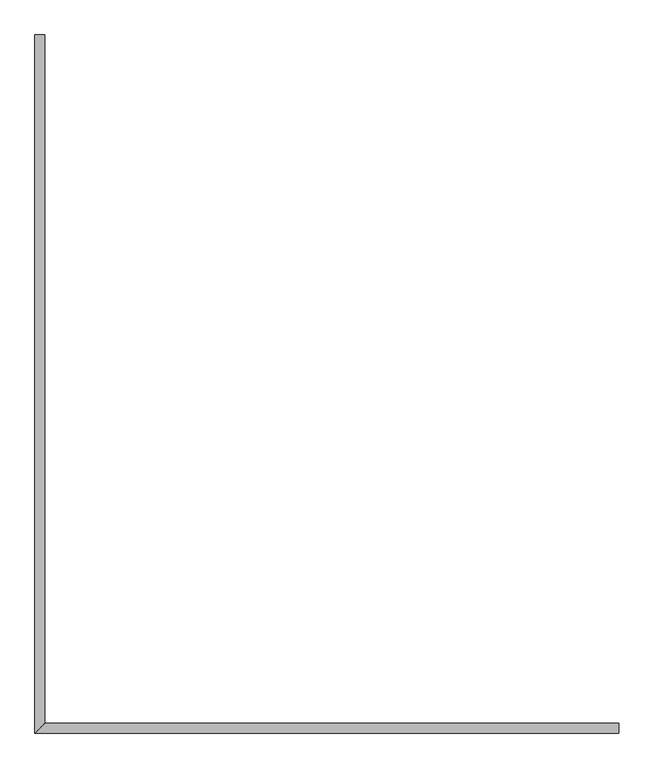
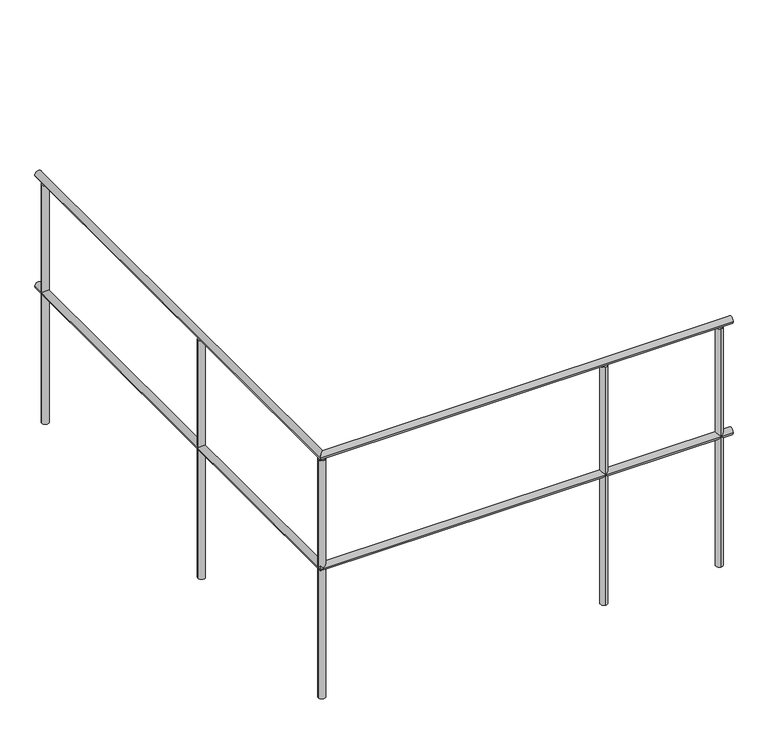
"""IFC4 building model written with IfcOpenShell, lengths in millimetres: railing geometry."""

from ifc_helpers import new_model, si_unit, point, frame, frame_2d, origin, place, context, project, spatial, circle_curve, ellipse_curve, trimmed, segment, composite_curve, outline, extrude, source, transform, mapped, element, save
from ifc_brep_helpers import plane_surface, cylinder_surface, advanced_brep


def railing_e5dc5f3b(model_context):
    return source(origin(), model_context, "Body", "SolidModel", [
        advanced_brep(
        [(-2206.0, 33046.2934796, 885.0), (-2176.0, 33046.2934796, 885.0), (-2176.0, 30976.2934796, 885.0), (-2206.0, 30946.2934796, 885.0), (-450.0, 30946.2934796, 885.0), (-450.0, 30976.2934796, 885.0)],
        [
            (0, 1, circle_curve(frame((-2191.0, 33046.2934796, 885.0), z_axis=(0.0, 1.0, 0.0), x_axis=(1.0, 0.0, 0.0)), 15.0)),
            (1, 0, circle_curve(frame((-2191.0, 33046.2934796, 885.0), z_axis=(0.0, 1.0, 0.0), x_axis=(1.0, 0.0, 0.0)), 15.0)),
            (1, 2),
            (2, 3, ellipse_curve(frame((-2191.0, 30961.2934796, 885.0), z_axis=(-0.707106781186546, 0.707106781186549, 0.0), x_axis=(0.7071067811865489, 0.707106781186546, 0.0)), 21.2132034, 15.0)),
            (3, 0),
            (3, 2, ellipse_curve(frame((-2191.0, 30961.2934796, 885.0), z_axis=(-0.707106781186546, 0.707106781186549, 0.0), x_axis=(0.7071067811865489, 0.707106781186546, 0.0)), 21.2132034, 15.0)),
            (4, 5, circle_curve(frame((-450.0, 30961.2934796, 885.0), z_axis=(1.0, 0.0, 0.0), x_axis=(0.0, 1.0, 0.0)), 15.0)),
            (5, 4, circle_curve(frame((-450.0, 30961.2934796, 885.0), z_axis=(1.0, 0.0, 0.0), x_axis=(0.0, 1.0, 0.0)), 15.0)),
            (2, 5),
            (4, 3),
        ],
        [
            plane_surface(frame((-2191.0, 33046.2934796, 900.0), z_axis=(0.0, 1.0, 0.0), x_axis=(0.0, 0.0, -1.0))),
            cylinder_surface(frame((-2191.0, 33046.2934796, 885.0), z_axis=(0.0, 1.0, 0.0), x_axis=(1.0, 0.0, 0.0)), 15.0),
            plane_surface(frame((-450.0, 30961.2934796, 900.0), z_axis=(1.0, 0.0, 0.0), x_axis=(0.0, 1.0, 0.0))),
            cylinder_surface(frame((-2191.0, 30961.2934796, 885.0), z_axis=(-1.0, 0.0, 0.0), x_axis=(0.0, 1.0, 0.0)), 15.0),
        ],
        [
            (0, [[1, 2]]),
            (1, [[-2, 3, 4, 5]]),
            (1, [[-1, -5, 6, -3]]),
            (2, [[7, 8]]),
            (3, [[-4, 9, -7, 10]]),
            (3, [[-6, -10, -8, -9]]),
        ],
    ),
        advanced_brep(
        [(-2206.0, 33046.2934796, 1385.0), (-2176.0, 33046.2934796, 1385.0), (-2176.0, 30976.2934796, 1385.0), (-2206.0, 30946.2934796, 1385.0), (-450.0, 30946.2934796, 1385.0), (-450.0, 30976.2934796, 1385.0)],
        [
            (0, 1, circle_curve(frame((-2191.0, 33046.2934796, 1385.0), z_axis=(0.0, 1.0, 0.0), x_axis=(1.0, 0.0, 0.0)), 15.0)),
            (1, 0, circle_curve(frame((-2191.0, 33046.2934796, 1385.0), z_axis=(0.0, 1.0, 0.0), x_axis=(1.0, 0.0, 0.0)), 15.0)),
            (1, 2),
            (2, 3, ellipse_curve(frame((-2191.0, 30961.2934796, 1385.0), z_axis=(-0.707106781186546, 0.707106781186549, 0.0), x_axis=(0.7071067811865489, 0.707106781186546, 0.0)), 21.2132034, 15.0)),
            (3, 0),
            (3, 2, ellipse_curve(frame((-2191.0, 30961.2934796, 1385.0), z_axis=(-0.707106781186546, 0.707106781186549, 0.0), x_axis=(0.7071067811865489, 0.707106781186546, 0.0)), 21.2132034, 15.0)),
            (4, 5, circle_curve(frame((-450.0, 30961.2934796, 1385.0), z_axis=(1.0, 0.0, 0.0), x_axis=(0.0, 1.0, 0.0)), 15.0)),
            (5, 4, circle_curve(frame((-450.0, 30961.2934796, 1385.0), z_axis=(1.0, 0.0, 0.0), x_axis=(0.0, 1.0, 0.0)), 15.0)),
            (2, 5),
            (4, 3),
        ],
        [
            plane_surface(frame((-2191.0, 33046.2934796, 1400.0), z_axis=(0.0, 1.0, 0.0), x_axis=(0.0, 0.0, -1.0))),
            cylinder_surface(frame((-2191.0, 33046.2934796, 1385.0), z_axis=(0.0, 1.0, 0.0), x_axis=(1.0, 0.0, 0.0)), 15.0),
            plane_surface(frame((-450.0, 30961.2934796, 1400.0), z_axis=(1.0, 0.0, 0.0), x_axis=(0.0, 1.0, 0.0))),
            cylinder_surface(frame((-2191.0, 30961.2934796, 1385.0), z_axis=(-1.0, 0.0, 0.0), x_axis=(0.0, 1.0, 0.0)), 15.0),
        ],
        [
            (0, [[1, 2]]),
            (1, [[-2, 3, 4, 5]]),
            (1, [[-1, -5, 6, -3]]),
            (2, [[7, 8]]),
            (3, [[-4, 9, -7, 10]]),
            (3, [[-6, -10, -8, -9]]),
        ],
    ),
        extrude(outline(composite_curve([segment(trimmed(circle_curve(frame_2d((-991.0, 30961.2934796)), 15.0), [point((-991.0, 30946.2934796))], [point((-991.0, 30976.2934796))], False, "CARTESIAN"), True, "CONTINUOUS"), segment(trimmed(circle_curve(frame_2d((-991.0, 30961.2934796)), 15.0), [point((-991.0, 30976.2934796))], [point((-991.0, 30946.2934796))], False, "CARTESIAN"), True, "CONTINUOUS")], self_intersect=False)), frame((0.0, 0.0, 300.0), z_axis=(0.0, 0.0, 1.0), x_axis=(1.0, 0.0, 0.0)), (0.0, 0.0, 1.0), 1070.0),
        extrude(outline(composite_curve([segment(trimmed(circle_curve(frame_2d((-2191.0, 31846.2934796)), 15.0), [point((-2206.0, 31846.2934796))], [point((-2176.0, 31846.2934796))], False, "CARTESIAN"), True, "CONTINUOUS"), segment(trimmed(circle_curve(frame_2d((-2191.0, 31846.2934796)), 15.0), [point((-2176.0, 31846.2934796))], [point((-2206.0, 31846.2934796))], False, "CARTESIAN"), True, "CONTINUOUS")], self_intersect=False)), frame((0.0, 0.0, 300.0), z_axis=(0.0, 0.0, 1.0), x_axis=(1.0, 0.0, 0.0)), (0.0, 0.0, 1.0), 1070.0),
        extrude(outline(composite_curve([segment(trimmed(circle_curve(frame_2d((-2191.0, 30961.2934796)), 15.0), [point((-2206.0, 30961.2934796))], [point((-2176.0, 30961.2934796))], False, "CARTESIAN"), True, "CONTINUOUS"), segment(trimmed(circle_curve(frame_2d((-2191.0, 30961.2934796)), 15.0), [point((-2176.0, 30961.2934796))], [point((-2206.0, 30961.2934796))], False, "CARTESIAN"), True, "CONTINUOUS")], self_intersect=False)), frame((0.0, 0.0, 300.0), z_axis=(0.0, 0.0, 1.0), x_axis=(1.0, 0.0, 0.0)), (0.0, 0.0, 1.0), 1070.0),
        extrude(outline(composite_curve([segment(trimmed(circle_curve(frame_2d((-500.0, 30961.2934796)), 15.0), [point((-500.0, 30946.2934796))], [point((-500.0, 30976.2934796))], False, "CARTESIAN"), True, "CONTINUOUS"), segment(trimmed(circle_curve(frame_2d((-500.0, 30961.2934796)), 15.0), [point((-500.0, 30976.2934796))], [point((-500.0, 30946.2934796))], False, "CARTESIAN"), True, "CONTINUOUS")], self_intersect=False)), frame((0.0, 0.0, 300.0), z_axis=(0.0, 0.0, 1.0), x_axis=(1.0, 0.0, 0.0)), (0.0, 0.0, 1.0), 1070.0),
        extrude(outline(composite_curve([segment(trimmed(circle_curve(frame_2d((-2191.0, 32996.2934796)), 15.0), [point((-2206.0, 32996.2934796))], [point((-2176.0, 32996.2934796))], False, "CARTESIAN"), True, "CONTINUOUS"), segment(trimmed(circle_curve(frame_2d((-2191.0, 32996.2934796)), 15.0), [point((-2176.0, 32996.2934796))], [point((-2206.0, 32996.2934796))], False, "CARTESIAN"), True, "CONTINUOUS")], self_intersect=False)), frame((0.0, 0.0, 300.0), z_axis=(0.0, 0.0, 1.0), x_axis=(1.0, 0.0, 0.0)), (0.0, 0.0, 1.0), 1070.0),
    ])


if __name__ == "__main__":
    model = new_model("IFC4")
    model_context = context("Model", 3, world=origin())
    ifc_project = project(units=[si_unit("LENGTHUNIT", "METRE", prefix="MILLI")], contexts=[model_context])
    site = spatial("IfcSite", under=ifc_project)
    building = spatial("IfcBuilding", under=site)
    placement = place(None, origin())
    railing_shape = railing_e5dc5f3b(model_context)
    element("IfcRailing", 1, at=placement, inside=building, context=model_context, shape_type="MappedRepresentation", body=[
        mapped(railing_shape, transform((0.0, 0.0, 0.0), x_axis=(1.0, 0.0, 0.0), y_axis=(0.0, 1.0, 0.0), z_axis=(0.0, 0.0, 1.0))),
    ])
    save(model, "model.ifc")
